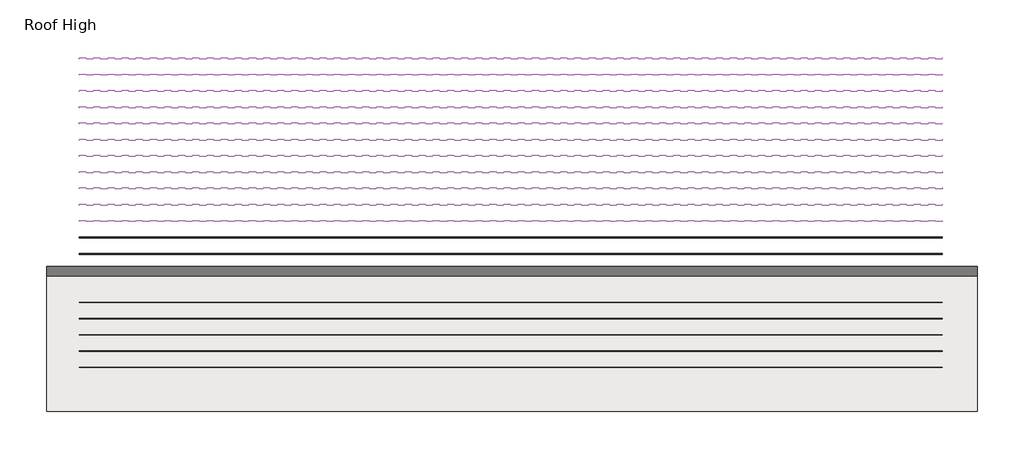
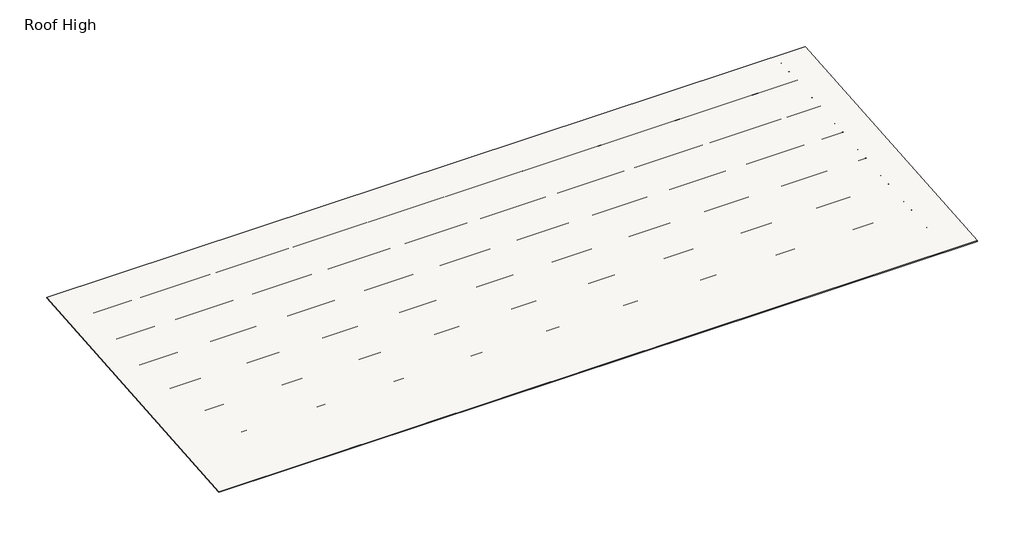
# One storey: 20 beams, 1 roof.
"""IFC4 building model written with IfcOpenShell, lengths in millimetres."""

import ifcopenshell
import ifcopenshell.guid

model = None  # the IFC model being written
_history = None  # IfcOwnerHistory: only IFC2X3 demands one
_inside = {}  # id of a spatial element -> (the spatial element, [elements in it])
_under = {}  # id of a project, library or spatial element -> (it, [spatial elements below it])
_declared = {}  # id of a project -> (the project, [libraries it declares])
_typed = {}  # id of a type object -> (the type object, [elements of that type])
_made_of = {}  # id of a material, layer set ... -> (it, [elements and type objects made of it])


def new_model(schema):
    """Start an empty IFC model of exactly this schema.

    Asked for "IFC4X3", IfcOpenShell would pick the latest addendum, in which some entities
    have other attributes; the version numbers below select the first issue.
    IFC2X3 requires an IfcOwnerHistory on every rooted entity: one is made here for all.
    """
    global model, _history
    if schema == "IFC4X3":
        model = ifcopenshell.file(schema_version=(4, 3, 0, 0))
    else:
        model = ifcopenshell.file(schema=schema)
    _inside.clear()
    _under.clear()
    _declared.clear()
    _typed.clear()
    _made_of.clear()
    _history = None
    if model.schema == "IFC2X3":
        org = make("IfcOrganization", Name="unknown")
        user = make(
            "IfcPersonAndOrganization",
            ThePerson=make("IfcPerson", FamilyName="unknown"),
            TheOrganization=org,
        )
        app = make(
            "IfcApplication",
            ApplicationDeveloper=org,
            Version="unknown",
            ApplicationFullName="unknown",
            ApplicationIdentifier="unknown",
        )
        _history = make(
            "IfcOwnerHistory",
            OwningUser=user,
            OwningApplication=app,
            ChangeAction="ADDED",
            CreationDate=0,
        )
    return model


def make(cls, **values):
    """One entity of the class cls with the attributes given. An attribute that is None is left unset."""
    return model.create_entity(
        cls, **{name: value for name, value in values.items() if value is not None}
    )


def rooted(cls, **values):
    """An entity with a GlobalId (a new one), such as an element, a storey or a relation."""
    return make(cls, GlobalId=ifcopenshell.guid.new(), OwnerHistory=_history, **values)


def si_unit(unit_type, name, prefix=None):
    """IfcSIUnit, for example si_unit("LENGTHUNIT", "METRE", prefix="MILLI")."""
    return make("IfcSIUnit", UnitType=unit_type, Prefix=prefix, Name=name)


def assignment(units):
    """IfcUnitAssignment: the units of a project."""
    return None if units is None else make("IfcUnitAssignment", Units=units)


def point(xyz):
    """IfcCartesianPoint."""
    return None if xyz is None else make("IfcCartesianPoint", Coordinates=xyz)


def direction(xyz):
    """IfcDirection."""
    return None if xyz is None else make("IfcDirection", DirectionRatios=xyz)


def frame(location, z_axis=None, x_axis=None):
    """IfcAxis2Placement3D, a coordinate frame: its origin and axes. An axis left out is left unset."""
    return make(
        "IfcAxis2Placement3D",
        Location=point(location),
        Axis=direction(z_axis),
        RefDirection=direction(x_axis),
    )


def frame_2d(location, x_axis=None):
    """IfcAxis2Placement2D, a coordinate frame in the plane: its origin and x axis."""
    return make(
        "IfcAxis2Placement2D", Location=point(location), RefDirection=direction(x_axis)
    )


def origin():
    """The frame at (0, 0, 0) with its axes left unset."""
    return frame((0.0, 0.0, 0.0))


def place(relative_to, where):
    """IfcLocalPlacement: puts the frame where relative to a parent placement (None: the world)."""
    return make(
        "IfcLocalPlacement", PlacementRelTo=relative_to, RelativePlacement=where
    )


def context(
    kind, dimensions, precision=None, world=None, true_north=None, identifier=None
):
    """IfcGeometricRepresentationContext, for example the 3D "Model" context."""
    return make(
        "IfcGeometricRepresentationContext",
        ContextIdentifier=identifier,
        ContextType=kind,
        CoordinateSpaceDimension=dimensions,
        Precision=precision,
        WorldCoordinateSystem=world,
        TrueNorth=true_north,
    )


def project(units=None, contexts=None):
    """IfcProject with its units and contexts."""
    return rooted(
        "IfcProject",
        Name="project",
        RepresentationContexts=contexts,
        UnitsInContext=assignment(units),
    )


def spatial(cls, under=None, at=None, **own):
    """A site, building, storey or space (cls), placed at a placement, below another one or the project."""
    s = rooted(cls, ObjectPlacement=at, **own)
    if under is not None:
        _under.setdefault(under.id(), (under, []))[1].append(s)
    return s


def polyline(points):
    """IfcPolyline through the points."""
    return make("IfcPolyline", Points=[point(p) for p in points])


def circle_curve(where, radius):
    """IfcCircle in the frame where."""
    return make("IfcCircle", Position=where, Radius=radius)


def trimmed(basis, trim1, trim2, sense, master):
    """IfcTrimmedCurve: the piece of a basis curve between two trims."""
    return make(
        "IfcTrimmedCurve",
        BasisCurve=basis,
        Trim1=trim1,
        Trim2=trim2,
        SenseAgreement=sense,
        MasterRepresentation=master,
    )


def segment(curve, same_sense, transition):
    """IfcCompositeCurveSegment."""
    return make(
        "IfcCompositeCurveSegment",
        Transition=transition,
        SameSense=same_sense,
        ParentCurve=curve,
    )


def composite_curve(segments, self_intersect=None):
    """IfcCompositeCurve: segments joined end to end."""
    return make("IfcCompositeCurve", Segments=segments, SelfIntersect=self_intersect)


def outline(outer, holes=None, kind="AREA"):
    """IfcArbitraryClosedProfileDef: a profile drawn as a closed curve; with holes, ...WithVoids."""
    if holes is None:
        return make("IfcArbitraryClosedProfileDef", ProfileType=kind, OuterCurve=outer)
    return make(
        "IfcArbitraryProfileDefWithVoids",
        ProfileType=kind,
        OuterCurve=outer,
        InnerCurves=holes,
    )


def extrude(swept, where, along, depth):
    """IfcExtrudedAreaSolid: the profile swept, set in the frame where, extruded along a direction by depth."""
    return make(
        "IfcExtrudedAreaSolid",
        SweptArea=swept,
        Position=where,
        ExtrudedDirection=direction(along),
        Depth=depth,
    )


def shape(context_of_items, identifier, shape_type, items):
    """IfcShapeRepresentation: the items that make up one representation, for example the "Body"."""
    return make(
        "IfcShapeRepresentation",
        ContextOfItems=context_of_items,
        RepresentationIdentifier=identifier,
        RepresentationType=shape_type,
        Items=items,
    )


def source(mapping_origin, context_of_items, identifier, shape_type, items):
    """IfcRepresentationMap: a shape defined once, which mapped items show again and again."""
    return make(
        "IfcRepresentationMap",
        MappingOrigin=mapping_origin,
        MappedRepresentation=shape(context_of_items, identifier, shape_type, items),
    )


def transform(
    local_origin,
    x_axis=None,
    y_axis=None,
    z_axis=None,
    scale=None,
    scale2=None,
    scale3=None,
    uniform=True,
):
    """IfcCartesianTransformationOperator3D, or its non-uniform kind. x_axis, y_axis, z_axis: its Axis1, 2, 3."""
    if uniform:
        return make(
            "IfcCartesianTransformationOperator3D",
            Axis1=direction(x_axis),
            Axis2=direction(y_axis),
            LocalOrigin=point(local_origin),
            Scale=scale,
            Axis3=direction(z_axis),
        )
    return make(
        "IfcCartesianTransformationOperator3DnonUniform",
        Axis1=direction(x_axis),
        Axis2=direction(y_axis),
        LocalOrigin=point(local_origin),
        Scale=scale,
        Axis3=direction(z_axis),
        Scale2=scale2,
        Scale3=scale3,
    )


def mapped(mapping_source, mapping_target):
    """IfcMappedItem: shows the shape of a source again, moved by a transform."""
    return make(
        "IfcMappedItem", MappingSource=mapping_source, MappingTarget=mapping_target
    )


def made_of(thing, what):
    """Note that an element or type object is made of a material, layer set ...; save() writes the relation."""
    if what is not None:
        _made_of.setdefault(what.id(), (what, []))[1].append(thing)
    return thing


def element(
    cls,
    number,
    at=None,
    inside=None,
    cuts=None,
    type_object=None,
    material=None,
    context=None,
    identifier="Body",
    shape_type=None,
    held_by="IfcProductDefinitionShape",
    body=None,
    shapes=None,
    **own,
):
    """One element of the class cls, such as IfcWall. Its Tag is "e" and its number.

    at: its placement. inside: the storey or other place that contains it. cuts: it is an
    opening in that element (IfcRelVoidsElement). A single representation is given by context,
    identifier, shape_type and body (its items); several are given by shapes. held_by: the class
    of the entity that holds the representations. save() writes the other relations.
    """
    e = rooted(cls, Tag="e%d" % number, ObjectPlacement=at, **own)
    if body is not None:
        shapes = [shape(context, identifier, shape_type, body)]
    if shapes is not None:
        e.Representation = make(held_by, Representations=shapes)
    if inside is not None:
        _inside.setdefault(inside.id(), (inside, []))[1].append(e)
    if cuts is not None:
        rooted(
            "IfcRelVoidsElement", RelatingBuildingElement=cuts, RelatedOpeningElement=e
        )
    if type_object is not None:
        _typed.setdefault(type_object.id(), (type_object, []))[1].append(e)
    return made_of(e, material)


def aggregate(whole, parts):
    """IfcRelAggregates: a whole, such as a stair, and the parts it consists of."""
    return rooted("IfcRelAggregates", RelatingObject=whole, RelatedObjects=parts)


def save(model, path):
    """Write the relations noted so far, then the file.

    IfcRelAggregates (storeys below a building ...), IfcRelContainedInSpatialStructure (elements
    in a storey), IfcRelDefinesByType, IfcRelAssociatesMaterial and IfcRelDeclares: one each for
    every whole, place, type object, material and project.
    """
    for whole, parts in _under.values():
        aggregate(whole, parts)
    for where, things in _inside.values():
        rooted(
            "IfcRelContainedInSpatialStructure",
            RelatedElements=things,
            RelatingStructure=where,
        )
    for kind, things in _typed.values():
        rooted("IfcRelDefinesByType", RelatedObjects=things, RelatingType=kind)
    for what, things in _made_of.values():
        rooted("IfcRelAssociatesMaterial", RelatedObjects=things, RelatingMaterial=what)
    for by, libraries in _declared.values():
        rooted("IfcRelDeclares", RelatingContext=by, RelatedDefinitions=libraries)
    model.write(path)


def beam_2a24e19f(model_context):
    return source(origin(), model_context, "Body", "SweptSolid", [
        extrude(outline(composite_curve([segment(polyline([(63.5, 127.0), (75.745104, 112.4068534), (73.6169367, 110.621109), (62.204539, 124.221875), (3.3005807, 124.221875)]), True, "CONTINUOUS"), segment(trimmed(circle_curve(frame_2d((3.3741066, 122.2381931)), 1.9850441), [point((3.3005807, 124.221875))], [point((1.3890625, 122.2381931))], True, "CARTESIAN"), True, "CONTINUOUS"), segment(polyline([(1.3890625, 122.2381931), (1.3890625, -122.2375)]), True, "CONTINUOUS"), segment(trimmed(circle_curve(frame_2d((-3.3734375, -122.2375)), 4.7625), [point((1.3890625, -122.2375))], [point((-3.3734375, -127.0))], False, "CARTESIAN"), True, "CONTINUOUS"), segment(polyline([(-3.3734375, -127.0), (-63.5, -127.0), (-75.745104, -112.4068534), (-73.6169367, -110.621109), (-62.204539, -124.221875), (-3.2694106, -124.221875)]), True, "CONTINUOUS"), segment(trimmed(circle_curve(frame_2d((-3.3748024, -122.2389339)), 1.9857399), [point((-3.2694106, -124.221875))], [point((-1.3890625, -122.2389339))], True, "CARTESIAN"), True, "CONTINUOUS"), segment(polyline([(-1.3890625, -122.2389339), (-1.3890625, 122.2375)]), True, "CONTINUOUS"), segment(trimmed(circle_curve(frame_2d((3.3734375, 122.2375)), 4.7625), [point((-1.3890625, 122.2375))], [point((3.3734375, 127.0))], False, "CARTESIAN"), True, "CONTINUOUS"), segment(polyline([(3.3734375, 127.0), (63.5, 127.0)]), True, "CONTINUOUS")], self_intersect=False)), frame((-40373.3, 0.0, 0.0), z_axis=(1.0, 0.0, 0.0), x_axis=(0.0, 1.0, 0.0)), (0.0, 0.0, 1.0), 80505.2999999),
    ])


model = new_model("IFC4")

# Units and contexts
model_context = context("Model", 3, world=origin())
ifc_project = project(units=[si_unit("LENGTHUNIT", "METRE", prefix="MILLI")], contexts=[model_context])

# Site, building, storey
site = spatial("IfcSite", under=ifc_project)
building = spatial("IfcBuilding", under=site)
storey = spatial("IfcBuildingStorey", under=building, Name="Roof High", Elevation=8432.8)

# Beams
placement = place(None, origin())
beam_shape = beam_2a24e19f(model_context)
element("IfcBeam", 1, ObjectType="Girt_Z : 10\"D", at=placement, inside=storey, context=model_context, shape_type="MappedRepresentation", body=[
    mapped(beam_shape, transform((619401.6117241, -537763.9066312, 11075.359772), x_axis=(1.0, 0.0, 0.0), y_axis=(0.0, 0.996545758244879, 0.08304547985374816), z_axis=(0.0, -0.08304547985374816, 0.996545758244879))),
])
element("IfcBeam", 2, ObjectType="Girt_Z : 10\"D", at=placement, inside=storey, context=model_context, shape_type="MappedRepresentation", body=[
    mapped(beam_shape, transform((619401.6117241, -539282.6423668, 10948.7984607), x_axis=(1.0, 0.0, 0.0), y_axis=(0.0, 0.996545758244879, 0.08304547985374816), z_axis=(0.0, -0.08304547985374816, 0.996545758244879))),
])
element("IfcBeam", 3, ObjectType="Girt_Z : 10\"D", at=placement, inside=storey, context=model_context, shape_type="MappedRepresentation", body=[
    mapped(beam_shape, transform((619401.6117241, -540801.3781023, 10822.2371494), x_axis=(1.0, 0.0, 0.0), y_axis=(0.0, 0.996545758244879, 0.08304547985374816), z_axis=(0.0, -0.08304547985374816, 0.996545758244879))),
])
element("IfcBeam", 4, ObjectType="Girt_Z : 10\"D", at=placement, inside=storey, context=model_context, shape_type="MappedRepresentation", body=[
    mapped(beam_shape, transform((619401.6117241, -542320.1138379, 10695.6758381), x_axis=(1.0, 0.0, 0.0), y_axis=(0.0, 0.996545758244879, 0.08304547985374816), z_axis=(0.0, -0.08304547985374816, 0.996545758244879))),
])
element("IfcBeam", 5, ObjectType="Girt_Z : 10\"D", at=placement, inside=storey, context=model_context, shape_type="MappedRepresentation", body=[
    mapped(beam_shape, transform((619401.6117241, -543838.8495735, 10569.1145268), x_axis=(1.0, 0.0, 0.0), y_axis=(0.0, 0.996545758244879, 0.08304547985374816), z_axis=(0.0, -0.08304547985374816, 0.996545758244879))),
])
element("IfcBeam", 6, ObjectType="Girt_Z : 10\"D", at=placement, inside=storey, context=model_context, shape_type="MappedRepresentation", body=[
    mapped(beam_shape, transform((619401.6117241, -545357.585309, 10442.5532155), x_axis=(1.0, 0.0, 0.0), y_axis=(0.0, 0.996545758244879, 0.08304547985374816), z_axis=(0.0, -0.08304547985374816, 0.996545758244879))),
])
element("IfcBeam", 7, ObjectType="Girt_Z : 10\"D", at=placement, inside=storey, context=model_context, shape_type="MappedRepresentation", body=[
    mapped(beam_shape, transform((619401.6117241, -546876.3210446, 10315.9919043), x_axis=(1.0, 0.0, 0.0), y_axis=(0.0, 0.996545758244879, 0.08304547985374816), z_axis=(0.0, -0.08304547985374816, 0.996545758244879))),
])
element("IfcBeam", 8, ObjectType="Girt_Z : 10\"D", at=placement, inside=storey, context=model_context, shape_type="MappedRepresentation", body=[
    mapped(beam_shape, transform((619401.6117241, -548395.0567802, 10189.430593), x_axis=(1.0, 0.0, 0.0), y_axis=(0.0, 0.996545758244879, 0.08304547985374816), z_axis=(0.0, -0.08304547985374816, 0.996545758244879))),
])
element("IfcBeam", 9, ObjectType="Girt_Z : 10\"D", at=placement, inside=storey, context=model_context, shape_type="MappedRepresentation", body=[
    mapped(beam_shape, transform((619401.6117241, -549913.7925157, 10062.8692817), x_axis=(1.0, 0.0, 0.0), y_axis=(0.0, 0.996545758244879, 0.08304547985374816), z_axis=(0.0, -0.08304547985374816, 0.996545758244879))),
])
element("IfcBeam", 10, ObjectType="Girt_Z : 10\"D", at=placement, inside=storey, context=model_context, shape_type="MappedRepresentation", body=[
    mapped(beam_shape, transform((619401.6117241, -551432.5282513, 9936.3079704), x_axis=(1.0, 0.0, 0.0), y_axis=(0.0, 0.996545758244879, 0.08304547985374816), z_axis=(0.0, -0.08304547985374816, 0.996545758244879))),
])
element("IfcBeam", 11, ObjectType="Girt_Z : 10\"D", at=placement, inside=storey, context=model_context, shape_type="MappedRepresentation", body=[
    mapped(beam_shape, transform((619401.6117241, -552951.2639869, 9809.7466591), x_axis=(1.0, 0.0, 0.0), y_axis=(0.0, 0.996545758244879, 0.08304547985374816), z_axis=(0.0, -0.08304547985374816, 0.996545758244879))),
])
element("IfcBeam", 12, ObjectType="Girt_Z : 10\"D", at=placement, inside=storey, context=model_context, shape_type="MappedRepresentation", body=[
    mapped(beam_shape, transform((619401.6117241, -554469.9997224, 9683.1853478), x_axis=(1.0, 0.0, 0.0), y_axis=(0.0, 0.996545758244879, 0.08304547985374816), z_axis=(0.0, -0.08304547985374816, 0.996545758244879))),
])
element("IfcBeam", 13, ObjectType="Girt_Z : 10\"D", at=placement, inside=storey, context=model_context, shape_type="MappedRepresentation", body=[
    mapped(beam_shape, transform((619401.6117241, -555988.735458, 9556.6240365), x_axis=(1.0, 0.0, 0.0), y_axis=(0.0, 0.996545758244879, 0.08304547985374816), z_axis=(0.0, -0.08304547985374816, 0.996545758244879))),
])
element("IfcBeam", 14, ObjectType="Girt_Z : 10\"D", at=placement, inside=storey, context=model_context, shape_type="MappedRepresentation", body=[
    mapped(beam_shape, transform((619401.6117241, -557507.4711936, 9430.0627252), x_axis=(1.0, 0.0, 0.0), y_axis=(0.0, 0.996545758244879, 0.08304547985374816), z_axis=(0.0, -0.08304547985374816, 0.996545758244879))),
])
element("IfcBeam", 15, ObjectType="Girt_Z : 10\"D", at=placement, inside=storey, context=model_context, shape_type="MappedRepresentation", body=[
    mapped(beam_shape, transform((619401.6117241, -559026.2069291, 9303.5014139), x_axis=(1.0, 0.0, 0.0), y_axis=(0.0, 0.996545758244879, 0.08304547985374816), z_axis=(0.0, -0.08304547985374816, 0.996545758244879))),
])
element("IfcBeam", 16, ObjectType="Girt_Z : 10\"D", at=placement, inside=storey, context=model_context, shape_type="MappedRepresentation", body=[
    mapped(beam_shape, transform((619401.6117241, -560544.9426647, 9176.9401026), x_axis=(1.0, 0.0, 0.0), y_axis=(0.0, 0.996545758244879, 0.08304547985374816), z_axis=(0.0, -0.08304547985374816, 0.996545758244879))),
])
element("IfcBeam", 17, ObjectType="Girt_Z : 10\"D", at=placement, inside=storey, context=model_context, shape_type="MappedRepresentation", body=[
    mapped(beam_shape, transform((619401.6117241, -562063.6784003, 9050.3787913), x_axis=(1.0, 0.0, 0.0), y_axis=(0.0, 0.996545758244879, 0.08304547985374816), z_axis=(0.0, -0.08304547985374816, 0.996545758244879))),
])
element("IfcBeam", 18, ObjectType="Girt_Z : 10\"D", at=placement, inside=storey, context=model_context, shape_type="MappedRepresentation", body=[
    mapped(beam_shape, transform((619401.6117241, -563582.4141358, 8923.81748), x_axis=(1.0, 0.0, 0.0), y_axis=(0.0, 0.996545758244879, 0.08304547985374816), z_axis=(0.0, -0.08304547985374816, 0.996545758244879))),
])
element("IfcBeam", 19, ObjectType="Girt_Z : 10\"D", at=placement, inside=storey, context=model_context, shape_type="MappedRepresentation", body=[
    mapped(beam_shape, transform((619401.6117241, -565101.1498714, 8797.2561687), x_axis=(1.0, 0.0, 0.0), y_axis=(0.0, 0.996545758244879, 0.08304547985374816), z_axis=(0.0, -0.08304547985374816, 0.996545758244879))),
])
element("IfcBeam", 20, ObjectType="Girt_Z : 10\"D", at=placement, inside=storey, context=model_context, shape_type="MappedRepresentation", body=[
    mapped(beam_shape, transform((619401.6117241, -566619.8856069, 8670.6948574), x_axis=(1.0, 0.0, 0.0), y_axis=(0.0, 0.996545758244879, 0.08304547985374816), z_axis=(0.0, -0.08304547985374816, 0.996545758244879))),
])

# Roof
element("IfcRoof", 21, ObjectType="Roof_High", at=placement, inside=storey, context=model_context, shape_type="SweptSolid", body=[
    extrude(outline(polyline([(-570739.3413841, 8582.1112108), (-536652.5413841, 11422.6778775), (-536652.5413841, 11346.2137519), (-570739.3413841, 8505.6470853), (-570739.3413841, 8582.1112108)])), frame((575980.3117239, 0.0, 0.0), z_axis=(1.0, 0.0, 0.0), x_axis=(0.0, 1.0, 0.0)), (0.0, 0.0, 1.0), 86842.6),
])

save(model, "model.ifc")

# Revit data of these elements
# Type "Girt_Z : 10\"D"
#   Web_Thickness = 0' - 0 7/64"
#   Length [instance default] = 10' - 0"
#   Leg_1 = 0' - 2 1/2"
#   Height = 0' - 10"
# Type "Roof_High"
#   Assembly Code = "B1020"
#   built-in parameter 1001600 = 0.25 (stored number, unit not read)
#   Layers, outside or top first: 0' - 3" no material (function 1)
# Elements 1, 2, 3, 4, 5, 6, 7, 8, 9, 10, 11, 12, 13, 14, 15, 16, 17, 18, 19, 20 (IfcBeam, "Girt_Z : 10\"D")
#   Phase Created = Phase 1
# Element 21 (IfcRoof, "Roof_High")
#   built-in parameter 1001705 = 37.476 (stored number, unit not read)
#   built-in parameter 1001701 = 0.239 (stored number, unit not read)
#   built-in parameter 1001710 = 33615
#   Phase Created = Phase 1
#   Materials on its faces: "Default Roof"
# Materials
#   "Default Roof": class "Miscellaneous", colour RGB 88 101 114, transparency 0
